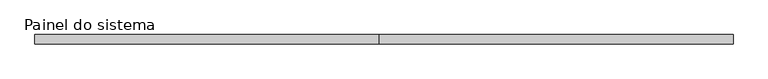
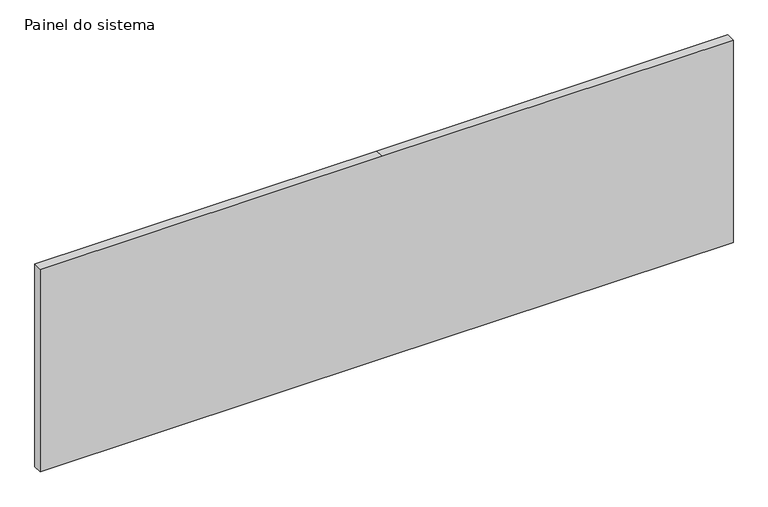
"""IFC4 building model written with IfcOpenShell, lengths in millimetres: plate geometry, Painel do sistema : Envidraçado."""

import ifcopenshell
import ifcopenshell.guid

model = None  # the IFC model being written
_history = None  # IfcOwnerHistory: only IFC2X3 demands one
_inside = {}  # id of a spatial element -> (the spatial element, [elements in it])
_under = {}  # id of a project, library or spatial element -> (it, [spatial elements below it])
_declared = {}  # id of a project -> (the project, [libraries it declares])
_typed = {}  # id of a type object -> (the type object, [elements of that type])
_made_of = {}  # id of a material, layer set ... -> (it, [elements and type objects made of it])


def new_model(schema):
    """Start an empty IFC model of exactly this schema.

    Asked for "IFC4X3", IfcOpenShell would pick the latest addendum, in which some entities
    have other attributes; the version numbers below select the first issue.
    IFC2X3 requires an IfcOwnerHistory on every rooted entity: one is made here for all.
    """
    global model, _history
    if schema == "IFC4X3":
        model = ifcopenshell.file(schema_version=(4, 3, 0, 0))
    else:
        model = ifcopenshell.file(schema=schema)
    _inside.clear()
    _under.clear()
    _declared.clear()
    _typed.clear()
    _made_of.clear()
    _history = None
    if model.schema == "IFC2X3":
        org = make("IfcOrganization", Name="unknown")
        user = make(
            "IfcPersonAndOrganization",
            ThePerson=make("IfcPerson", FamilyName="unknown"),
            TheOrganization=org,
        )
        app = make(
            "IfcApplication",
            ApplicationDeveloper=org,
            Version="unknown",
            ApplicationFullName="unknown",
            ApplicationIdentifier="unknown",
        )
        _history = make(
            "IfcOwnerHistory",
            OwningUser=user,
            OwningApplication=app,
            ChangeAction="ADDED",
            CreationDate=0,
        )
    return model


def make(cls, **values):
    """One entity of the class cls with the attributes given. An attribute that is None is left unset."""
    return model.create_entity(
        cls, **{name: value for name, value in values.items() if value is not None}
    )


def rooted(cls, **values):
    """An entity with a GlobalId (a new one), such as an element, a storey or a relation."""
    return make(cls, GlobalId=ifcopenshell.guid.new(), OwnerHistory=_history, **values)


def si_unit(unit_type, name, prefix=None):
    """IfcSIUnit, for example si_unit("LENGTHUNIT", "METRE", prefix="MILLI")."""
    return make("IfcSIUnit", UnitType=unit_type, Prefix=prefix, Name=name)


def assignment(units):
    """IfcUnitAssignment: the units of a project."""
    return None if units is None else make("IfcUnitAssignment", Units=units)


def point(xyz):
    """IfcCartesianPoint."""
    return None if xyz is None else make("IfcCartesianPoint", Coordinates=xyz)


def direction(xyz):
    """IfcDirection."""
    return None if xyz is None else make("IfcDirection", DirectionRatios=xyz)


def frame(location, z_axis=None, x_axis=None):
    """IfcAxis2Placement3D, a coordinate frame: its origin and axes. An axis left out is left unset."""
    return make(
        "IfcAxis2Placement3D",
        Location=point(location),
        Axis=direction(z_axis),
        RefDirection=direction(x_axis),
    )


def origin():
    """The frame at (0, 0, 0) with its axes left unset."""
    return frame((0.0, 0.0, 0.0))


def place(relative_to, where):
    """IfcLocalPlacement: puts the frame where relative to a parent placement (None: the world)."""
    return make(
        "IfcLocalPlacement", PlacementRelTo=relative_to, RelativePlacement=where
    )


def context(
    kind, dimensions, precision=None, world=None, true_north=None, identifier=None
):
    """IfcGeometricRepresentationContext, for example the 3D "Model" context."""
    return make(
        "IfcGeometricRepresentationContext",
        ContextIdentifier=identifier,
        ContextType=kind,
        CoordinateSpaceDimension=dimensions,
        Precision=precision,
        WorldCoordinateSystem=world,
        TrueNorth=true_north,
    )


def project(units=None, contexts=None):
    """IfcProject with its units and contexts."""
    return rooted(
        "IfcProject",
        Name="project",
        RepresentationContexts=contexts,
        UnitsInContext=assignment(units),
    )


def spatial(cls, under=None, at=None, **own):
    """A site, building, storey or space (cls), placed at a placement, below another one or the project."""
    s = rooted(cls, ObjectPlacement=at, **own)
    if under is not None:
        _under.setdefault(under.id(), (under, []))[1].append(s)
    return s


def polyline(points):
    """IfcPolyline through the points."""
    return make("IfcPolyline", Points=[point(p) for p in points])


def outline(outer, holes=None, kind="AREA"):
    """IfcArbitraryClosedProfileDef: a profile drawn as a closed curve; with holes, ...WithVoids."""
    if holes is None:
        return make("IfcArbitraryClosedProfileDef", ProfileType=kind, OuterCurve=outer)
    return make(
        "IfcArbitraryProfileDefWithVoids",
        ProfileType=kind,
        OuterCurve=outer,
        InnerCurves=holes,
    )


def extrude(swept, where, along, depth):
    """IfcExtrudedAreaSolid: the profile swept, set in the frame where, extruded along a direction by depth."""
    return make(
        "IfcExtrudedAreaSolid",
        SweptArea=swept,
        Position=where,
        ExtrudedDirection=direction(along),
        Depth=depth,
    )


def shape(context_of_items, identifier, shape_type, items):
    """IfcShapeRepresentation: the items that make up one representation, for example the "Body"."""
    return make(
        "IfcShapeRepresentation",
        ContextOfItems=context_of_items,
        RepresentationIdentifier=identifier,
        RepresentationType=shape_type,
        Items=items,
    )


def source(mapping_origin, context_of_items, identifier, shape_type, items):
    """IfcRepresentationMap: a shape defined once, which mapped items show again and again."""
    return make(
        "IfcRepresentationMap",
        MappingOrigin=mapping_origin,
        MappedRepresentation=shape(context_of_items, identifier, shape_type, items),
    )


def transform(
    local_origin,
    x_axis=None,
    y_axis=None,
    z_axis=None,
    scale=None,
    scale2=None,
    scale3=None,
    uniform=True,
):
    """IfcCartesianTransformationOperator3D, or its non-uniform kind. x_axis, y_axis, z_axis: its Axis1, 2, 3."""
    if uniform:
        return make(
            "IfcCartesianTransformationOperator3D",
            Axis1=direction(x_axis),
            Axis2=direction(y_axis),
            LocalOrigin=point(local_origin),
            Scale=scale,
            Axis3=direction(z_axis),
        )
    return make(
        "IfcCartesianTransformationOperator3DnonUniform",
        Axis1=direction(x_axis),
        Axis2=direction(y_axis),
        LocalOrigin=point(local_origin),
        Scale=scale,
        Axis3=direction(z_axis),
        Scale2=scale2,
        Scale3=scale3,
    )


def mapped(mapping_source, mapping_target):
    """IfcMappedItem: shows the shape of a source again, moved by a transform."""
    return make(
        "IfcMappedItem", MappingSource=mapping_source, MappingTarget=mapping_target
    )


def made_of(thing, what):
    """Note that an element or type object is made of a material, layer set ...; save() writes the relation."""
    if what is not None:
        _made_of.setdefault(what.id(), (what, []))[1].append(thing)
    return thing


def element(
    cls,
    number,
    at=None,
    inside=None,
    cuts=None,
    type_object=None,
    material=None,
    context=None,
    identifier="Body",
    shape_type=None,
    held_by="IfcProductDefinitionShape",
    body=None,
    shapes=None,
    **own,
):
    """One element of the class cls, such as IfcWall. Its Tag is "e" and its number.

    at: its placement. inside: the storey or other place that contains it. cuts: it is an
    opening in that element (IfcRelVoidsElement). A single representation is given by context,
    identifier, shape_type and body (its items); several are given by shapes. held_by: the class
    of the entity that holds the representations. save() writes the other relations.
    """
    e = rooted(cls, Tag="e%d" % number, ObjectPlacement=at, **own)
    if body is not None:
        shapes = [shape(context, identifier, shape_type, body)]
    if shapes is not None:
        e.Representation = make(held_by, Representations=shapes)
    if inside is not None:
        _inside.setdefault(inside.id(), (inside, []))[1].append(e)
    if cuts is not None:
        rooted(
            "IfcRelVoidsElement", RelatingBuildingElement=cuts, RelatedOpeningElement=e
        )
    if type_object is not None:
        _typed.setdefault(type_object.id(), (type_object, []))[1].append(e)
    return made_of(e, material)


def aggregate(whole, parts):
    """IfcRelAggregates: a whole, such as a stair, and the parts it consists of."""
    return rooted("IfcRelAggregates", RelatingObject=whole, RelatedObjects=parts)


def save(model, path):
    """Write the relations noted so far, then the file.

    IfcRelAggregates (storeys below a building ...), IfcRelContainedInSpatialStructure (elements
    in a storey), IfcRelDefinesByType, IfcRelAssociatesMaterial and IfcRelDeclares: one each for
    every whole, place, type object, material and project.
    """
    for whole, parts in _under.values():
        aggregate(whole, parts)
    for where, things in _inside.values():
        rooted(
            "IfcRelContainedInSpatialStructure",
            RelatedElements=things,
            RelatingStructure=where,
        )
    for kind, things in _typed.values():
        rooted("IfcRelDefinesByType", RelatedObjects=things, RelatingType=kind)
    for what, things in _made_of.values():
        rooted("IfcRelAssociatesMaterial", RelatedObjects=things, RelatingMaterial=what)
    for by, libraries in _declared.values():
        rooted("IfcRelDeclares", RelatingContext=by, RelatedDefinitions=libraries)
    model.write(path)


def painel_do_sistema_b3a4ee0d(model_context):
    return source(origin(), model_context, "Body", "SweptSolid", [
        extrude(outline(polyline([(0.0, -954.2100001), (0.0, -12.4999998), (0.0, 954.2100001), (590.0, 954.2100001), (590.0, -12.4999998), (590.0, -954.2100001), (0.0, -954.2100001)])), frame((0.0, -49.5, 0.0), z_axis=(0.0, 1.0, 0.0), x_axis=(0.0, 0.0, 1.0)), (0.0, 0.0, 1.0), 25.0),
    ])


if __name__ == "__main__":
    model = new_model("IFC4")
    model_context = context("Model", 3, world=origin())
    ifc_project = project(units=[si_unit("LENGTHUNIT", "METRE", prefix="MILLI")], contexts=[model_context])
    site = spatial("IfcSite", under=ifc_project)
    building = spatial("IfcBuilding", under=site)
    placement = place(None, origin())
    painel_do_sistema_shape = painel_do_sistema_b3a4ee0d(model_context)
    element("IfcPlate", 1, ObjectType="Painel do sistema : Envidraçado", at=placement, inside=building, context=model_context, shape_type="MappedRepresentation", body=[
        mapped(painel_do_sistema_shape, transform((0.0, 0.0, 0.0), x_axis=(1.0, 0.0, 0.0), y_axis=(0.0, 1.0, 0.0), z_axis=(0.0, 0.0, 1.0))),
    ])
    save(model, "model.ifc")

# Revit data of these elements
# Type "Painel do sistema : Envidraçado"
#   Construction Type Id = "GSP4R"
#   Analytic Construction = "Vidraça única Pilkington 1/8 pol"
#   Visual Light Transmittance = 0.9
#   Solar Heat Gain Coefficient = 0.86
#   Heat Transfer Coefficient (U) = 6.7069 W/(m²·K)
# Element 1 (IfcPlate, "Painel do sistema : Envidraçado")
#   Materials on its faces: ".VIDRO GENÉRICO"
# Materials
#   ".VIDRO GENÉRICO": class ".CC_VIDRO", colour RGB 0 128 192, transparency 0.9, Description = "Vidro comum", Cost = 0
